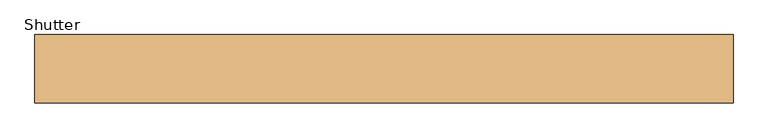
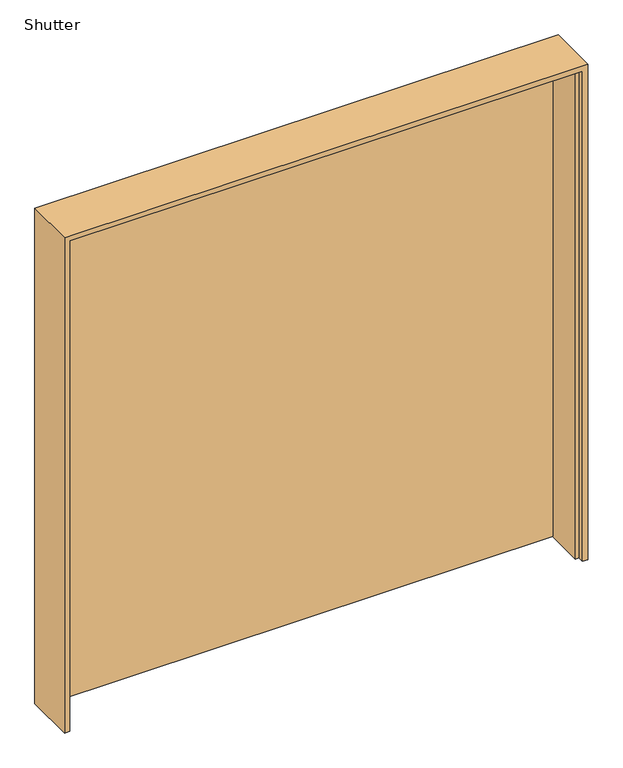
"""IFC4 building model written with IfcOpenShell, lengths in millimetres: door geometry, Shutter : H_DR_AMB_Roll up Door_Steel_W3000xH3000_Motorized."""

from ifc_helpers import new_model, si_unit, origin, origin_with_axes, place, context, project, spatial, polyline, outline, extrude, faceted_brep, source, transform, mapped, element, save


def shutter_a73fe604(model_context):
    return source(origin(), model_context, "Body", "SolidModel", [
        extrude(outline(polyline([(1470.0, 147.0), (1470.0, 112.0), (-1470.0, 112.0), (-1470.0, 147.0), (1470.0, 147.0)])), origin_with_axes(), (0.0, 0.0, 1.0), 2970.0),
        faceted_brep([(1470.0, 147.0, 0.0), (1500.0, 147.0, 0.0), (1500.0, -147.0, 0.0), (1470.0, -147.0, 0.0), (1470.0, -112.0, 0.0), (1450.0, -112.0, 0.0), (1450.0, 112.0, 0.0), (1470.0, 112.0, 0.0), (1470.0, 147.0, 2970.0), (-1470.0, 147.0, 2970.0), (-1470.0, 147.0, 0.0), (-1500.0, 147.0, 0.0), (-1500.0, 147.0, 3000.0), (1500.0, 147.0, 3000.0), (1500.0, -147.0, 3000.0), (-1500.0, -147.0, 3000.0), (-1500.0, -147.0, 0.0), (-1470.0, -147.0, 0.0), (-1470.0, -147.0, 2970.0), (1470.0, -147.0, 2970.0), (1470.0, -112.0, 2970.0), (-1470.0, -112.0, 2970.0), (-1470.0, -112.0, 0.0), (-1450.0, -112.0, 0.0), (-1450.0, -112.0, 2950.0), (1450.0, -112.0, 2950.0), (1450.0, 112.0, 2950.0), (-1450.0, 112.0, 2950.0), (-1450.0, 112.0, 0.0), (-1470.0, 112.0, 0.0), (-1470.0, 112.0, 2970.0), (1470.0, 112.0, 2970.0)], [[[0, 1, 2, 3, 4, 5, 6, 7]], [[1, 0, 8, 9, 10, 11, 12, 13]], [[2, 1, 13, 14]], [[3, 2, 14, 15, 16, 17, 18, 19]], [[4, 3, 19, 20]], [[5, 4, 20, 21, 22, 23, 24, 25]], [[6, 5, 25, 26]], [[7, 6, 26, 27, 28, 29, 30, 31]], [[0, 7, 31, 8]], [[9, 30, 29, 10]], [[10, 29, 28, 23, 22, 17, 16, 11]], [[15, 12, 11, 16]], [[21, 18, 17, 22]], [[27, 24, 23, 28]], [[8, 31, 30, 9]], [[14, 13, 12, 15]], [[20, 19, 18, 21]], [[26, 25, 24, 27]]]),
    ])


if __name__ == "__main__":
    model = new_model("IFC4")
    model_context = context("Model", 3, world=origin())
    ifc_project = project(units=[si_unit("LENGTHUNIT", "METRE", prefix="MILLI")], contexts=[model_context])
    site = spatial("IfcSite", under=ifc_project)
    building = spatial("IfcBuilding", under=site)
    placement = place(None, origin())
    shutter_shape = shutter_a73fe604(model_context)
    element("IfcDoor", 1, ObjectType="Shutter : H_DR_AMB_Roll up Door_Steel_W3000xH3000_Motorized", at=placement, inside=building, context=model_context, shape_type="MappedRepresentation", body=[
        mapped(shutter_shape, transform((0.0, 0.0, 0.0), x_axis=(1.0, 0.0, 0.0), y_axis=(0.0, 1.0, 0.0), z_axis=(0.0, 0.0, 1.0))),
    ])
    save(model, "model.ifc")

# Revit data of these elements
# Type "Shutter : H_DR_AMB_Roll up Door_Steel_W3000xH3000_Motorized"
#   Type Mark = "364"
#   Analytic Construction = "<None>"
#   프레임 투영 외부. = 25 mm
#   프레임 투영 내부. = 25 mm
#   프레임 폭 = 75 mm
#   Height = 3000 mm
#   Width = 3000 mm
#   Define Thermal Properties by = 1
#   문 패널 = none
#   문 프레임 = none
#   Function = (empty or 0)
#   Wall Closure = (empty or 0)
